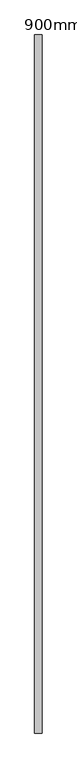
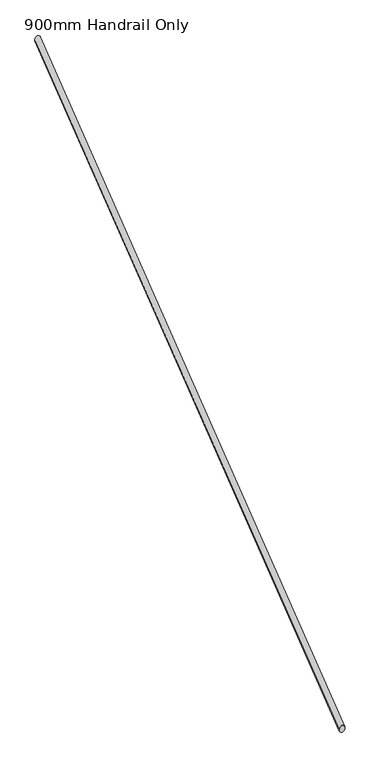
"""IFC4 building model written with IfcOpenShell, lengths in millimetres: railing geometry, 900mm Handrail Only."""

from ifc_helpers import new_model, si_unit, frame, origin, place, context, project, spatial, ellipse_curve, source, transform, mapped, element, save
from ifc_brep_helpers import plane_surface, cylinder_surface, advanced_brep


def railing_900mm_handrail_only_0678b89a(model_context):
    return source(origin(), model_context, "Body", "AdvancedBrep", [
        advanced_brep(
        [(8338.0, -11825.0, 1068.4468381), (8378.0, -11825.0, 1068.4468381), (8338.0, -8075.0, 3974.6968381), (8378.0, -8075.0, 3974.6968381)],
        [
            (0, 1, ellipse_curve(frame((8358.0, -11825.0, 1068.4468381), z_axis=(0.0, -1.0, 0.0), x_axis=(0.0, 0.0, -1.0)), 25.3031619, 20.0)),
            (1, 0, ellipse_curve(frame((8358.0, -11825.0, 1068.4468381), z_axis=(0.0, -1.0, 0.0), x_axis=(0.0, 0.0, -1.0)), 25.3031619, 20.0)),
            (2, 3, ellipse_curve(frame((8358.0, -8075.0, 3974.6968381), z_axis=(0.0, 1.0, 0.0), x_axis=(0.0, 0.0, -1.0)), 25.3031619, 20.0)),
            (3, 2, ellipse_curve(frame((8358.0, -8075.0, 3974.6968381), z_axis=(0.0, 1.0, 0.0), x_axis=(0.0, 0.0, -1.0)), 25.3031619, 20.0)),
            (0, 2),
            (3, 1),
        ],
        [
            plane_surface(frame((8358.0, -11825.0, 1093.75), z_axis=(0.0, -1.0, 0.0), x_axis=(0.0, 0.0, 1.0))),
            plane_surface(frame((8358.0, -8075.0, 4000.0), z_axis=(0.0, 1.0, 0.0), x_axis=(0.0, 0.0, 1.0))),
            cylinder_surface(frame((8358.0, -11812.7485667, 1077.941699), z_axis=(0.0, -0.7904150521752251, -0.612571665435838), x_axis=(1.0, 0.0, 0.0)), 20.0),
        ],
        [
            (0, [[1, 2]]),
            (1, [[3, 4]]),
            (2, [[-1, 5, -4, 6]]),
            (2, [[-2, -6, -3, -5]]),
        ],
    ),
    ])


if __name__ == "__main__":
    model = new_model("IFC4")
    model_context = context("Model", 3, world=origin())
    ifc_project = project(units=[si_unit("LENGTHUNIT", "METRE", prefix="MILLI")], contexts=[model_context])
    site = spatial("IfcSite", under=ifc_project)
    building = spatial("IfcBuilding", under=site)
    placement = place(None, origin())
    railing_900mm_handrail_only_shape = railing_900mm_handrail_only_0678b89a(model_context)
    element("IfcRailing", 1, ObjectType="900mm Handrail Only", at=placement, inside=building, context=model_context, shape_type="MappedRepresentation", body=[
        mapped(railing_900mm_handrail_only_shape, transform((0.0, 0.0, 0.0), x_axis=(1.0, 0.0, 0.0), y_axis=(0.0, 1.0, 0.0), z_axis=(0.0, 0.0, 1.0))),
    ])
    save(model, "model.ifc")
